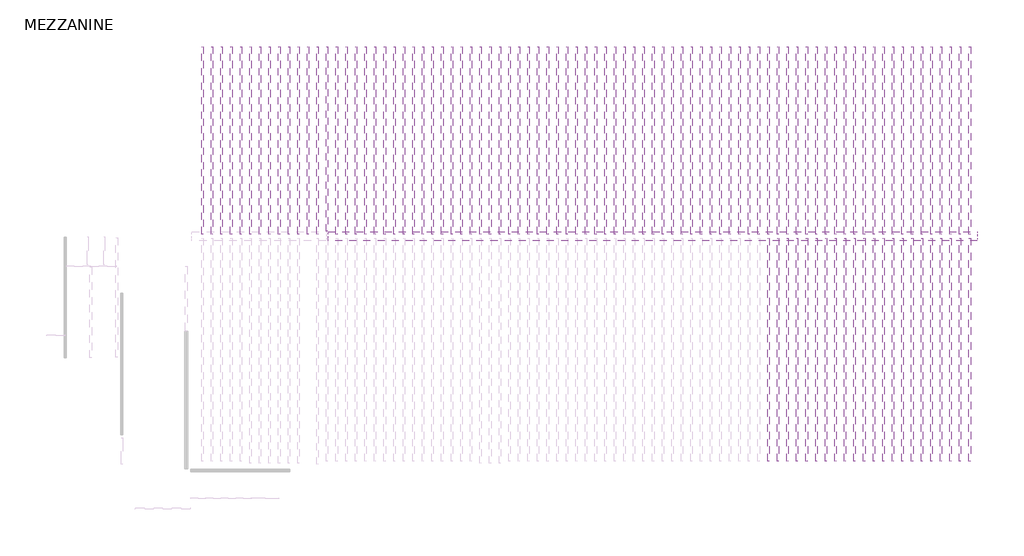
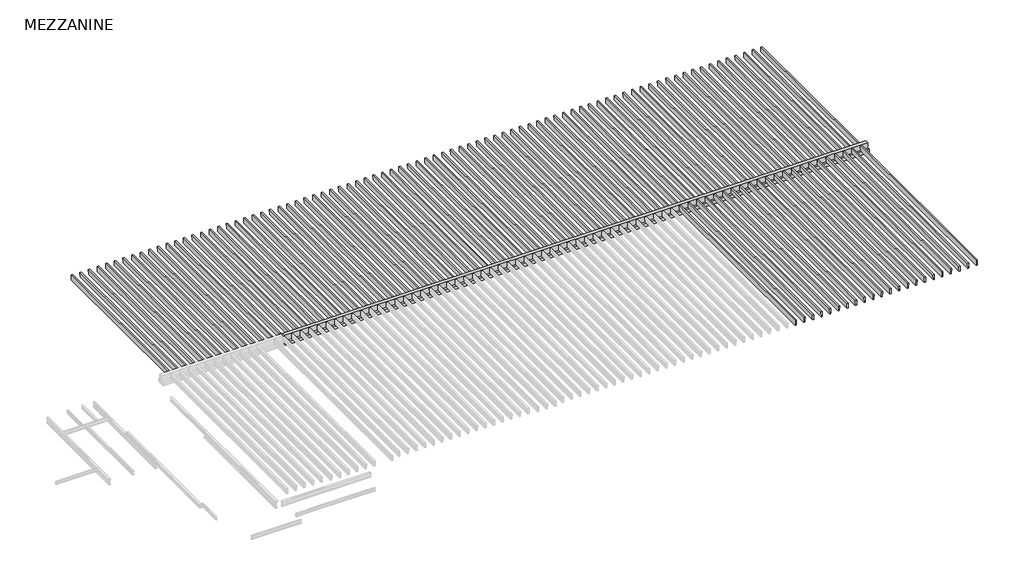
# One storey, part 2 of 2: 104 beams.
"""IFC4 building model written with IfcOpenShell, lengths in millimetres."""

import ifcopenshell
import ifcopenshell.guid

model = None  # the IFC model being written
_history = None  # IfcOwnerHistory: only IFC2X3 demands one
_inside = {}  # id of a spatial element -> (the spatial element, [elements in it])
_under = {}  # id of a project, library or spatial element -> (it, [spatial elements below it])
_declared = {}  # id of a project -> (the project, [libraries it declares])
_typed = {}  # id of a type object -> (the type object, [elements of that type])
_made_of = {}  # id of a material, layer set ... -> (it, [elements and type objects made of it])


def new_model(schema):
    """Start an empty IFC model of exactly this schema.

    Asked for "IFC4X3", IfcOpenShell would pick the latest addendum, in which some entities
    have other attributes; the version numbers below select the first issue.
    IFC2X3 requires an IfcOwnerHistory on every rooted entity: one is made here for all.
    """
    global model, _history
    if schema == "IFC4X3":
        model = ifcopenshell.file(schema_version=(4, 3, 0, 0))
    else:
        model = ifcopenshell.file(schema=schema)
    _inside.clear()
    _under.clear()
    _declared.clear()
    _typed.clear()
    _made_of.clear()
    _history = None
    if model.schema == "IFC2X3":
        org = make("IfcOrganization", Name="unknown")
        user = make(
            "IfcPersonAndOrganization",
            ThePerson=make("IfcPerson", FamilyName="unknown"),
            TheOrganization=org,
        )
        app = make(
            "IfcApplication",
            ApplicationDeveloper=org,
            Version="unknown",
            ApplicationFullName="unknown",
            ApplicationIdentifier="unknown",
        )
        _history = make(
            "IfcOwnerHistory",
            OwningUser=user,
            OwningApplication=app,
            ChangeAction="ADDED",
            CreationDate=0,
        )
    return model


def make(cls, **values):
    """One entity of the class cls with the attributes given. An attribute that is None is left unset."""
    return model.create_entity(
        cls, **{name: value for name, value in values.items() if value is not None}
    )


def rooted(cls, **values):
    """An entity with a GlobalId (a new one), such as an element, a storey or a relation."""
    return make(cls, GlobalId=ifcopenshell.guid.new(), OwnerHistory=_history, **values)


def si_unit(unit_type, name, prefix=None):
    """IfcSIUnit, for example si_unit("LENGTHUNIT", "METRE", prefix="MILLI")."""
    return make("IfcSIUnit", UnitType=unit_type, Prefix=prefix, Name=name)


def assignment(units):
    """IfcUnitAssignment: the units of a project."""
    return None if units is None else make("IfcUnitAssignment", Units=units)


def point(xyz):
    """IfcCartesianPoint."""
    return None if xyz is None else make("IfcCartesianPoint", Coordinates=xyz)


def direction(xyz):
    """IfcDirection."""
    return None if xyz is None else make("IfcDirection", DirectionRatios=xyz)


def frame(location, z_axis=None, x_axis=None):
    """IfcAxis2Placement3D, a coordinate frame: its origin and axes. An axis left out is left unset."""
    return make(
        "IfcAxis2Placement3D",
        Location=point(location),
        Axis=direction(z_axis),
        RefDirection=direction(x_axis),
    )


def origin():
    """The frame at (0, 0, 0) with its axes left unset."""
    return frame((0.0, 0.0, 0.0))


def place(relative_to, where):
    """IfcLocalPlacement: puts the frame where relative to a parent placement (None: the world)."""
    return make(
        "IfcLocalPlacement", PlacementRelTo=relative_to, RelativePlacement=where
    )


def context(
    kind, dimensions, precision=None, world=None, true_north=None, identifier=None
):
    """IfcGeometricRepresentationContext, for example the 3D "Model" context."""
    return make(
        "IfcGeometricRepresentationContext",
        ContextIdentifier=identifier,
        ContextType=kind,
        CoordinateSpaceDimension=dimensions,
        Precision=precision,
        WorldCoordinateSystem=world,
        TrueNorth=true_north,
    )


def project(units=None, contexts=None):
    """IfcProject with its units and contexts."""
    return rooted(
        "IfcProject",
        Name="project",
        RepresentationContexts=contexts,
        UnitsInContext=assignment(units),
    )


def spatial(cls, under=None, at=None, **own):
    """A site, building, storey or space (cls), placed at a placement, below another one or the project."""
    s = rooted(cls, ObjectPlacement=at, **own)
    if under is not None:
        _under.setdefault(under.id(), (under, []))[1].append(s)
    return s


def polyline(points):
    """IfcPolyline through the points."""
    return make("IfcPolyline", Points=[point(p) for p in points])


def outline(outer, holes=None, kind="AREA"):
    """IfcArbitraryClosedProfileDef: a profile drawn as a closed curve; with holes, ...WithVoids."""
    if holes is None:
        return make("IfcArbitraryClosedProfileDef", ProfileType=kind, OuterCurve=outer)
    return make(
        "IfcArbitraryProfileDefWithVoids",
        ProfileType=kind,
        OuterCurve=outer,
        InnerCurves=holes,
    )


def extrude(swept, where, along, depth):
    """IfcExtrudedAreaSolid: the profile swept, set in the frame where, extruded along a direction by depth."""
    return make(
        "IfcExtrudedAreaSolid",
        SweptArea=swept,
        Position=where,
        ExtrudedDirection=direction(along),
        Depth=depth,
    )


def shape(context_of_items, identifier, shape_type, items):
    """IfcShapeRepresentation: the items that make up one representation, for example the "Body"."""
    return make(
        "IfcShapeRepresentation",
        ContextOfItems=context_of_items,
        RepresentationIdentifier=identifier,
        RepresentationType=shape_type,
        Items=items,
    )


def source(mapping_origin, context_of_items, identifier, shape_type, items):
    """IfcRepresentationMap: a shape defined once, which mapped items show again and again."""
    return make(
        "IfcRepresentationMap",
        MappingOrigin=mapping_origin,
        MappedRepresentation=shape(context_of_items, identifier, shape_type, items),
    )


def transform(
    local_origin,
    x_axis=None,
    y_axis=None,
    z_axis=None,
    scale=None,
    scale2=None,
    scale3=None,
    uniform=True,
):
    """IfcCartesianTransformationOperator3D, or its non-uniform kind. x_axis, y_axis, z_axis: its Axis1, 2, 3."""
    if uniform:
        return make(
            "IfcCartesianTransformationOperator3D",
            Axis1=direction(x_axis),
            Axis2=direction(y_axis),
            LocalOrigin=point(local_origin),
            Scale=scale,
            Axis3=direction(z_axis),
        )
    return make(
        "IfcCartesianTransformationOperator3DnonUniform",
        Axis1=direction(x_axis),
        Axis2=direction(y_axis),
        LocalOrigin=point(local_origin),
        Scale=scale,
        Axis3=direction(z_axis),
        Scale2=scale2,
        Scale3=scale3,
    )


def mapped(mapping_source, mapping_target):
    """IfcMappedItem: shows the shape of a source again, moved by a transform."""
    return make(
        "IfcMappedItem", MappingSource=mapping_source, MappingTarget=mapping_target
    )


def made_of(thing, what):
    """Note that an element or type object is made of a material, layer set ...; save() writes the relation."""
    if what is not None:
        _made_of.setdefault(what.id(), (what, []))[1].append(thing)
    return thing


def element(
    cls,
    number,
    at=None,
    inside=None,
    cuts=None,
    type_object=None,
    material=None,
    context=None,
    identifier="Body",
    shape_type=None,
    held_by="IfcProductDefinitionShape",
    body=None,
    shapes=None,
    **own,
):
    """One element of the class cls, such as IfcWall. Its Tag is "e" and its number.

    at: its placement. inside: the storey or other place that contains it. cuts: it is an
    opening in that element (IfcRelVoidsElement). A single representation is given by context,
    identifier, shape_type and body (its items); several are given by shapes. held_by: the class
    of the entity that holds the representations. save() writes the other relations.
    """
    e = rooted(cls, Tag="e%d" % number, ObjectPlacement=at, **own)
    if body is not None:
        shapes = [shape(context, identifier, shape_type, body)]
    if shapes is not None:
        e.Representation = make(held_by, Representations=shapes)
    if inside is not None:
        _inside.setdefault(inside.id(), (inside, []))[1].append(e)
    if cuts is not None:
        rooted(
            "IfcRelVoidsElement", RelatingBuildingElement=cuts, RelatedOpeningElement=e
        )
    if type_object is not None:
        _typed.setdefault(type_object.id(), (type_object, []))[1].append(e)
    return made_of(e, material)


def aggregate(whole, parts):
    """IfcRelAggregates: a whole, such as a stair, and the parts it consists of."""
    return rooted("IfcRelAggregates", RelatingObject=whole, RelatedObjects=parts)


def save(model, path):
    """Write the relations noted so far, then the file.

    IfcRelAggregates (storeys below a building ...), IfcRelContainedInSpatialStructure (elements
    in a storey), IfcRelDefinesByType, IfcRelAssociatesMaterial and IfcRelDeclares: one each for
    every whole, place, type object, material and project.
    """
    for whole, parts in _under.values():
        aggregate(whole, parts)
    for where, things in _inside.values():
        rooted(
            "IfcRelContainedInSpatialStructure",
            RelatedElements=things,
            RelatingStructure=where,
        )
    for kind, things in _typed.values():
        rooted("IfcRelDefinesByType", RelatedObjects=things, RelatingType=kind)
    for what, things in _made_of.values():
        rooted("IfcRelAssociatesMaterial", RelatedObjects=things, RelatingMaterial=what)
    for by, libraries in _declared.values():
        rooted("IfcRelDeclares", RelatingContext=by, RelatedDefinitions=libraries)
    model.write(path)


def precast_cone_shaped_beam_double_t_c0c18137(model_context):
    return source(origin(), model_context, "Body", "SweptSolid", [
        extrude(outline(polyline([(50.8, -228.6), (-50.8, -228.6), (-63.5, 228.6), (63.5, 228.6), (50.8, -228.6)])), frame((-7378.7, 0.0, 0.0), z_axis=(1.0, 0.0, 0.0), x_axis=(0.0, 1.0, 0.0)), (0.0, 0.0, 1.0), 14909.8),
    ])


def precast_cone_shaped_beam_double_t_e9a1f935(model_context):
    return source(origin(), model_context, "Body", "SweptSolid", [
        extrude(outline(polyline([(50.8, -228.6), (-50.8, -228.6), (-63.5, 228.6), (63.5, 228.6), (50.8, -228.6)])), frame((-7162.8, 0.0, 0.0), z_axis=(1.0, 0.0, 0.0), x_axis=(0.0, 1.0, 0.0)), (0.0, 0.0, 1.0), 14693.9),
    ])


def precast_cone_shaped_beam_double_t_b6a0bb25(model_context):
    return source(origin(), model_context, "Body", "SweptSolid", [
        extrude(outline(polyline([(-50.8, -228.6), (-63.5, 228.6), (63.5, 228.6), (50.8, -228.6), (-50.8, -228.6)])), frame((-8915.4, 0.0, 0.0), z_axis=(1.0, 0.0, 0.0), x_axis=(0.0, 1.0, 0.0)), (0.0, 0.0, 1.0), 17741.9),
    ])


def precast_inverted_tee_20_12x28_ea35af0b(model_context):
    return source(origin(), model_context, "Body", "SweptSolid", [
        extrude(outline(polyline([(-355.6, -406.4), (-355.6, -101.6), (-152.4, -101.6), (-152.4, 406.4), (152.4, 406.4), (152.4, -101.6), (355.6, -101.6), (355.6, -406.4), (-355.6, -406.4)])), frame((-25831.8, 0.0, 0.0), z_axis=(1.0, 0.0, 0.0), x_axis=(0.0, 1.0, 0.0)), (0.0, 0.0, 1.0), 51587.4),
    ])


model = new_model("IFC4")

# Units and contexts
model_context = context("Model", 3, world=origin())
ifc_project = project(units=[si_unit("LENGTHUNIT", "METRE", prefix="MILLI")], contexts=[model_context])

# Site, building, storey
site = spatial("IfcSite", under=ifc_project)
building = spatial("IfcBuilding", under=site)
storey = spatial("IfcBuildingStorey", under=building, Name="MEZZANINE", Elevation=2959.1)

# Beams
placement = place(None, origin())
precast_cone_shaped_beam_double_t_shape = precast_cone_shaped_beam_double_t_c0c18137(model_context)
element("IfcBeam", 1, ObjectType="Precast-Cone Shaped Beam : DOUBLE_T", at=placement, inside=storey, context=model_context, shape_type="MappedRepresentation", body=[
    mapped(precast_cone_shaped_beam_double_t_shape, transform((-23461.5909443, 5367.0768471, 4724.4), x_axis=(0.0, 1.0, 0.0), y_axis=(-1.0, 0.0, 0.0), z_axis=(0.0, 0.0, 1.0))),
])
element("IfcBeam", 2, ObjectType="Precast-Cone Shaped Beam : DOUBLE_T", at=placement, inside=storey, context=model_context, shape_type="MappedRepresentation", body=[
    mapped(precast_cone_shaped_beam_double_t_shape, transform((-22699.5909443, 5367.0768471, 4724.4), x_axis=(0.0, 1.0, 0.0), y_axis=(-1.0, 0.0, 0.0), z_axis=(0.0, 0.0, 1.0))),
])
element("IfcBeam", 3, ObjectType="Precast-Cone Shaped Beam : DOUBLE_T", at=placement, inside=storey, context=model_context, shape_type="MappedRepresentation", body=[
    mapped(precast_cone_shaped_beam_double_t_shape, transform((-21937.5909443, 5367.0768471, 4724.4), x_axis=(0.0, 1.0, 0.0), y_axis=(-1.0, 0.0, 0.0), z_axis=(0.0, 0.0, 1.0))),
])
element("IfcBeam", 4, ObjectType="Precast-Cone Shaped Beam : DOUBLE_T", at=placement, inside=storey, context=model_context, shape_type="MappedRepresentation", body=[
    mapped(precast_cone_shaped_beam_double_t_shape, transform((-21175.5909443, 5367.0768471, 4724.4), x_axis=(0.0, 1.0, 0.0), y_axis=(-1.0, 0.0, 0.0), z_axis=(0.0, 0.0, 1.0))),
])
element("IfcBeam", 5, ObjectType="Precast-Cone Shaped Beam : DOUBLE_T", at=placement, inside=storey, context=model_context, shape_type="MappedRepresentation", body=[
    mapped(precast_cone_shaped_beam_double_t_shape, transform((-20413.5909443, 5367.0768471, 4724.4), x_axis=(0.0, 1.0, 0.0), y_axis=(-1.0, 0.0, 0.0), z_axis=(0.0, 0.0, 1.0))),
])
element("IfcBeam", 6, ObjectType="Precast-Cone Shaped Beam : DOUBLE_T", at=placement, inside=storey, context=model_context, shape_type="MappedRepresentation", body=[
    mapped(precast_cone_shaped_beam_double_t_shape, transform((-19651.5909443, 5367.0768471, 4724.4), x_axis=(0.0, 1.0, 0.0), y_axis=(-1.0, 0.0, 0.0), z_axis=(0.0, 0.0, 1.0))),
])
element("IfcBeam", 7, ObjectType="Precast-Cone Shaped Beam : DOUBLE_T", at=placement, inside=storey, context=model_context, shape_type="MappedRepresentation", body=[
    mapped(precast_cone_shaped_beam_double_t_shape, transform((-18889.5909443, 5367.0768471, 4724.4), x_axis=(0.0, 1.0, 0.0), y_axis=(-1.0, 0.0, 0.0), z_axis=(0.0, 0.0, 1.0))),
])
element("IfcBeam", 8, ObjectType="Precast-Cone Shaped Beam : DOUBLE_T", at=placement, inside=storey, context=model_context, shape_type="MappedRepresentation", body=[
    mapped(precast_cone_shaped_beam_double_t_shape, transform((-18127.5909443, 5367.0768471, 4724.4), x_axis=(0.0, 1.0, 0.0), y_axis=(-1.0, 0.0, 0.0), z_axis=(0.0, 0.0, 1.0))),
])
element("IfcBeam", 9, ObjectType="Precast-Cone Shaped Beam : DOUBLE_T", at=placement, inside=storey, context=model_context, shape_type="MappedRepresentation", body=[
    mapped(precast_cone_shaped_beam_double_t_shape, transform((-17365.5909443, 5367.0768471, 4724.4), x_axis=(0.0, 1.0, 0.0), y_axis=(-1.0, 0.0, 0.0), z_axis=(0.0, 0.0, 1.0))),
])
element("IfcBeam", 10, ObjectType="Precast-Cone Shaped Beam : DOUBLE_T", at=placement, inside=storey, context=model_context, shape_type="MappedRepresentation", body=[
    mapped(precast_cone_shaped_beam_double_t_shape, transform((-16603.5909443, 5367.0768471, 4724.4), x_axis=(0.0, 1.0, 0.0), y_axis=(-1.0, 0.0, 0.0), z_axis=(0.0, 0.0, 1.0))),
])
element("IfcBeam", 11, ObjectType="Precast-Cone Shaped Beam : DOUBLE_T", at=placement, inside=storey, context=model_context, shape_type="MappedRepresentation", body=[
    mapped(precast_cone_shaped_beam_double_t_shape, transform((-15841.5909443, 5367.0768471, 4724.4), x_axis=(0.0, 1.0, 0.0), y_axis=(-1.0, 0.0, 0.0), z_axis=(0.0, 0.0, 1.0))),
])
element("IfcBeam", 12, ObjectType="Precast-Cone Shaped Beam : DOUBLE_T", at=placement, inside=storey, context=model_context, shape_type="MappedRepresentation", body=[
    mapped(precast_cone_shaped_beam_double_t_shape, transform((-15079.5909443, 5367.0768471, 4724.4), x_axis=(0.0, 1.0, 0.0), y_axis=(-1.0, 0.0, 0.0), z_axis=(0.0, 0.0, 1.0))),
])
element("IfcBeam", 13, ObjectType="Precast-Cone Shaped Beam : DOUBLE_T", at=placement, inside=storey, context=model_context, shape_type="MappedRepresentation", body=[
    mapped(precast_cone_shaped_beam_double_t_shape, transform((-14317.5909443, 5367.0768471, 4724.4), x_axis=(0.0, 1.0, 0.0), y_axis=(-1.0, 0.0, 0.0), z_axis=(0.0, 0.0, 1.0))),
])
element("IfcBeam", 14, ObjectType="Precast-Cone Shaped Beam : DOUBLE_T", at=placement, inside=storey, context=model_context, shape_type="MappedRepresentation", body=[
    mapped(precast_cone_shaped_beam_double_t_shape, transform((-13555.5909443, 5367.0768471, 4724.4), x_axis=(0.0, 1.0, 0.0), y_axis=(-1.0, 0.0, 0.0), z_axis=(0.0, 0.0, 1.0))),
])
element("IfcBeam", 15, ObjectType="Precast-Cone Shaped Beam : DOUBLE_T", at=placement, inside=storey, context=model_context, shape_type="MappedRepresentation", body=[
    mapped(precast_cone_shaped_beam_double_t_shape, transform((-12793.5909443, 5367.0768471, 4724.4), x_axis=(0.0, 1.0, 0.0), y_axis=(-1.0, 0.0, 0.0), z_axis=(0.0, 0.0, 1.0))),
])
element("IfcBeam", 16, ObjectType="Precast-Cone Shaped Beam : DOUBLE_T", at=placement, inside=storey, context=model_context, shape_type="MappedRepresentation", body=[
    mapped(precast_cone_shaped_beam_double_t_shape, transform((-12031.5909443, 5367.0768471, 4724.4), x_axis=(0.0, 1.0, 0.0), y_axis=(-1.0, 0.0, 0.0), z_axis=(0.0, 0.0, 1.0))),
])
element("IfcBeam", 17, ObjectType="Precast-Cone Shaped Beam : DOUBLE_T", at=placement, inside=storey, context=model_context, shape_type="MappedRepresentation", body=[
    mapped(precast_cone_shaped_beam_double_t_shape, transform((-11269.5909443, 5367.0768471, 4724.4), x_axis=(0.0, 1.0, 0.0), y_axis=(-1.0, 0.0, 0.0), z_axis=(0.0, 0.0, 1.0))),
])
element("IfcBeam", 18, ObjectType="Precast-Cone Shaped Beam : DOUBLE_T", at=placement, inside=storey, context=model_context, shape_type="MappedRepresentation", body=[
    mapped(precast_cone_shaped_beam_double_t_shape, transform((-10507.5909443, 5367.0768471, 4724.4), x_axis=(0.0, 1.0, 0.0), y_axis=(-1.0, 0.0, 0.0), z_axis=(0.0, 0.0, 1.0))),
])
element("IfcBeam", 19, ObjectType="Precast-Cone Shaped Beam : DOUBLE_T", at=placement, inside=storey, context=model_context, shape_type="MappedRepresentation", body=[
    mapped(precast_cone_shaped_beam_double_t_shape, transform((-9745.5909443, 5367.0768471, 4724.4), x_axis=(0.0, 1.0, 0.0), y_axis=(-1.0, 0.0, 0.0), z_axis=(0.0, 0.0, 1.0))),
])
element("IfcBeam", 20, ObjectType="Precast-Cone Shaped Beam : DOUBLE_T", at=placement, inside=storey, context=model_context, shape_type="MappedRepresentation", body=[
    mapped(precast_cone_shaped_beam_double_t_shape, transform((-8983.5909443, 5367.0768471, 4724.4), x_axis=(0.0, 1.0, 0.0), y_axis=(-1.0, 0.0, 0.0), z_axis=(0.0, 0.0, 1.0))),
])
element("IfcBeam", 21, ObjectType="Precast-Cone Shaped Beam : DOUBLE_T", at=placement, inside=storey, context=model_context, shape_type="MappedRepresentation", body=[
    mapped(precast_cone_shaped_beam_double_t_shape, transform((-8221.5909443, 5367.0768471, 4724.4), x_axis=(0.0, 1.0, 0.0), y_axis=(-1.0, 0.0, 0.0), z_axis=(0.0, 0.0, 1.0))),
])
element("IfcBeam", 22, ObjectType="Precast-Cone Shaped Beam : DOUBLE_T", at=placement, inside=storey, context=model_context, shape_type="MappedRepresentation", body=[
    mapped(precast_cone_shaped_beam_double_t_shape, transform((-7459.5909443, 5367.0768471, 4724.4), x_axis=(0.0, 1.0, 0.0), y_axis=(-1.0, 0.0, 0.0), z_axis=(0.0, 0.0, 1.0))),
])
element("IfcBeam", 23, ObjectType="Precast-Cone Shaped Beam : DOUBLE_T", at=placement, inside=storey, context=model_context, shape_type="MappedRepresentation", body=[
    mapped(precast_cone_shaped_beam_double_t_shape, transform((-6697.5909443, 5367.0768471, 4724.4), x_axis=(0.0, 1.0, 0.0), y_axis=(-1.0, 0.0, 0.0), z_axis=(0.0, 0.0, 1.0))),
])
element("IfcBeam", 24, ObjectType="Precast-Cone Shaped Beam : DOUBLE_T", at=placement, inside=storey, context=model_context, shape_type="MappedRepresentation", body=[
    mapped(precast_cone_shaped_beam_double_t_shape, transform((-5935.5909443, 5367.0768471, 4724.4), x_axis=(0.0, 1.0, 0.0), y_axis=(-1.0, 0.0, 0.0), z_axis=(0.0, 0.0, 1.0))),
])
element("IfcBeam", 25, ObjectType="Precast-Cone Shaped Beam : DOUBLE_T", at=placement, inside=storey, context=model_context, shape_type="MappedRepresentation", body=[
    mapped(precast_cone_shaped_beam_double_t_shape, transform((-5173.5909443, 5367.0768471, 4724.4), x_axis=(0.0, 1.0, 0.0), y_axis=(-1.0, 0.0, 0.0), z_axis=(0.0, 0.0, 1.0))),
])
element("IfcBeam", 26, ObjectType="Precast-Cone Shaped Beam : DOUBLE_T", at=placement, inside=storey, context=model_context, shape_type="MappedRepresentation", body=[
    mapped(precast_cone_shaped_beam_double_t_shape, transform((-4411.5909443, 5367.0768471, 4724.4), x_axis=(0.0, 1.0, 0.0), y_axis=(-1.0, 0.0, 0.0), z_axis=(0.0, 0.0, 1.0))),
])
element("IfcBeam", 27, ObjectType="Precast-Cone Shaped Beam : DOUBLE_T", at=placement, inside=storey, context=model_context, shape_type="MappedRepresentation", body=[
    mapped(precast_cone_shaped_beam_double_t_shape, transform((-3649.5909443, 5367.0768471, 4724.4), x_axis=(0.0, 1.0, 0.0), y_axis=(-1.0, 0.0, 0.0), z_axis=(0.0, 0.0, 1.0))),
])
element("IfcBeam", 28, ObjectType="Precast-Cone Shaped Beam : DOUBLE_T", at=placement, inside=storey, context=model_context, shape_type="MappedRepresentation", body=[
    mapped(precast_cone_shaped_beam_double_t_shape, transform((-2887.5909443, 5367.0768471, 4724.4), x_axis=(0.0, 1.0, 0.0), y_axis=(-1.0, 0.0, 0.0), z_axis=(0.0, 0.0, 1.0))),
])
element("IfcBeam", 29, ObjectType="Precast-Cone Shaped Beam : DOUBLE_T", at=placement, inside=storey, context=model_context, shape_type="MappedRepresentation", body=[
    mapped(precast_cone_shaped_beam_double_t_shape, transform((-2125.5909443, 5367.0768471, 4724.4), x_axis=(0.0, 1.0, 0.0), y_axis=(-1.0, 0.0, 0.0), z_axis=(0.0, 0.0, 1.0))),
])
element("IfcBeam", 30, ObjectType="Precast-Cone Shaped Beam : DOUBLE_T", at=placement, inside=storey, context=model_context, shape_type="MappedRepresentation", body=[
    mapped(precast_cone_shaped_beam_double_t_shape, transform((-1363.5909443, 5367.0768471, 4724.4), x_axis=(0.0, 1.0, 0.0), y_axis=(-1.0, 0.0, 0.0), z_axis=(0.0, 0.0, 1.0))),
])
element("IfcBeam", 31, ObjectType="Precast-Cone Shaped Beam : DOUBLE_T", at=placement, inside=storey, context=model_context, shape_type="MappedRepresentation", body=[
    mapped(precast_cone_shaped_beam_double_t_shape, transform((-601.5909443, 5367.0768471, 4724.4), x_axis=(0.0, 1.0, 0.0), y_axis=(-1.0, 0.0, 0.0), z_axis=(0.0, 0.0, 1.0))),
])
element("IfcBeam", 32, ObjectType="Precast-Cone Shaped Beam : DOUBLE_T", at=placement, inside=storey, context=model_context, shape_type="MappedRepresentation", body=[
    mapped(precast_cone_shaped_beam_double_t_shape, transform((160.4090557, 5367.0768471, 4724.4), x_axis=(0.0, 1.0, 0.0), y_axis=(-1.0, 0.0, 0.0), z_axis=(0.0, 0.0, 1.0))),
])
element("IfcBeam", 33, ObjectType="Precast-Cone Shaped Beam : DOUBLE_T", at=placement, inside=storey, context=model_context, shape_type="MappedRepresentation", body=[
    mapped(precast_cone_shaped_beam_double_t_shape, transform((922.4090557, 5367.0768471, 4724.4), x_axis=(0.0, 1.0, 0.0), y_axis=(-1.0, 0.0, 0.0), z_axis=(0.0, 0.0, 1.0))),
])
element("IfcBeam", 34, ObjectType="Precast-Cone Shaped Beam : DOUBLE_T", at=placement, inside=storey, context=model_context, shape_type="MappedRepresentation", body=[
    mapped(precast_cone_shaped_beam_double_t_shape, transform((1684.4090557, 5367.0768471, 4724.4), x_axis=(0.0, 1.0, 0.0), y_axis=(-1.0, 0.0, 0.0), z_axis=(0.0, 0.0, 1.0))),
])
element("IfcBeam", 35, ObjectType="Precast-Cone Shaped Beam : DOUBLE_T", at=placement, inside=storey, context=model_context, shape_type="MappedRepresentation", body=[
    mapped(precast_cone_shaped_beam_double_t_shape, transform((2446.4090557, 5367.0768471, 4724.4), x_axis=(0.0, 1.0, 0.0), y_axis=(-1.0, 0.0, 0.0), z_axis=(0.0, 0.0, 1.0))),
])
element("IfcBeam", 36, ObjectType="Precast-Cone Shaped Beam : DOUBLE_T", at=placement, inside=storey, context=model_context, shape_type="MappedRepresentation", body=[
    mapped(precast_cone_shaped_beam_double_t_shape, transform((3208.4090557, 5367.0768471, 4724.4), x_axis=(0.0, 1.0, 0.0), y_axis=(-1.0, 0.0, 0.0), z_axis=(0.0, 0.0, 1.0))),
])
element("IfcBeam", 37, ObjectType="Precast-Cone Shaped Beam : DOUBLE_T", at=placement, inside=storey, context=model_context, shape_type="MappedRepresentation", body=[
    mapped(precast_cone_shaped_beam_double_t_shape, transform((3970.4090557, 5367.0768471, 4724.4), x_axis=(0.0, 1.0, 0.0), y_axis=(-1.0, 0.0, 0.0), z_axis=(0.0, 0.0, 1.0))),
])
element("IfcBeam", 38, ObjectType="Precast-Cone Shaped Beam : DOUBLE_T", at=placement, inside=storey, context=model_context, shape_type="MappedRepresentation", body=[
    mapped(precast_cone_shaped_beam_double_t_shape, transform((4732.4090557, 5367.0768471, 4724.4), x_axis=(0.0, 1.0, 0.0), y_axis=(-1.0, 0.0, 0.0), z_axis=(0.0, 0.0, 1.0))),
])
element("IfcBeam", 39, ObjectType="Precast-Cone Shaped Beam : DOUBLE_T", at=placement, inside=storey, context=model_context, shape_type="MappedRepresentation", body=[
    mapped(precast_cone_shaped_beam_double_t_shape, transform((5494.4090557, 5367.0768471, 4724.4), x_axis=(0.0, 1.0, 0.0), y_axis=(-1.0, 0.0, 0.0), z_axis=(0.0, 0.0, 1.0))),
])
element("IfcBeam", 40, ObjectType="Precast-Cone Shaped Beam : DOUBLE_T", at=placement, inside=storey, context=model_context, shape_type="MappedRepresentation", body=[
    mapped(precast_cone_shaped_beam_double_t_shape, transform((6256.4090557, 5367.0768471, 4724.4), x_axis=(0.0, 1.0, 0.0), y_axis=(-1.0, 0.0, 0.0), z_axis=(0.0, 0.0, 1.0))),
])
element("IfcBeam", 41, ObjectType="Precast-Cone Shaped Beam : DOUBLE_T", at=placement, inside=storey, context=model_context, shape_type="MappedRepresentation", body=[
    mapped(precast_cone_shaped_beam_double_t_shape, transform((7018.4090557, 5367.0768471, 4724.4), x_axis=(0.0, 1.0, 0.0), y_axis=(-1.0, 0.0, 0.0), z_axis=(0.0, 0.0, 1.0))),
])
element("IfcBeam", 42, ObjectType="Precast-Cone Shaped Beam : DOUBLE_T", at=placement, inside=storey, context=model_context, shape_type="MappedRepresentation", body=[
    mapped(precast_cone_shaped_beam_double_t_shape, transform((7780.4090557, 5367.0768471, 4724.4), x_axis=(0.0, 1.0, 0.0), y_axis=(-1.0, 0.0, 0.0), z_axis=(0.0, 0.0, 1.0))),
])
element("IfcBeam", 43, ObjectType="Precast-Cone Shaped Beam : DOUBLE_T", at=placement, inside=storey, context=model_context, shape_type="MappedRepresentation", body=[
    mapped(precast_cone_shaped_beam_double_t_shape, transform((8542.4090557, 5367.0768471, 4724.4), x_axis=(0.0, 1.0, 0.0), y_axis=(-1.0, 0.0, 0.0), z_axis=(0.0, 0.0, 1.0))),
])
element("IfcBeam", 44, ObjectType="Precast-Cone Shaped Beam : DOUBLE_T", at=placement, inside=storey, context=model_context, shape_type="MappedRepresentation", body=[
    mapped(precast_cone_shaped_beam_double_t_shape, transform((9304.4090557, 5367.0768471, 4724.4), x_axis=(0.0, 1.0, 0.0), y_axis=(-1.0, 0.0, 0.0), z_axis=(0.0, 0.0, 1.0))),
])
element("IfcBeam", 45, ObjectType="Precast-Cone Shaped Beam : DOUBLE_T", at=placement, inside=storey, context=model_context, shape_type="MappedRepresentation", body=[
    mapped(precast_cone_shaped_beam_double_t_shape, transform((10066.4090557, 5367.0768471, 4724.4), x_axis=(0.0, 1.0, 0.0), y_axis=(-1.0, 0.0, 0.0), z_axis=(0.0, 0.0, 1.0))),
])
element("IfcBeam", 46, ObjectType="Precast-Cone Shaped Beam : DOUBLE_T", at=placement, inside=storey, context=model_context, shape_type="MappedRepresentation", body=[
    mapped(precast_cone_shaped_beam_double_t_shape, transform((10828.4090557, 5367.0768471, 4724.4), x_axis=(0.0, 1.0, 0.0), y_axis=(-1.0, 0.0, 0.0), z_axis=(0.0, 0.0, 1.0))),
])
element("IfcBeam", 47, ObjectType="Precast-Cone Shaped Beam : DOUBLE_T", at=placement, inside=storey, context=model_context, shape_type="MappedRepresentation", body=[
    mapped(precast_cone_shaped_beam_double_t_shape, transform((11590.4090557, 5367.0768471, 4724.4), x_axis=(0.0, 1.0, 0.0), y_axis=(-1.0, 0.0, 0.0), z_axis=(0.0, 0.0, 1.0))),
])
element("IfcBeam", 48, ObjectType="Precast-Cone Shaped Beam : DOUBLE_T", at=placement, inside=storey, context=model_context, shape_type="MappedRepresentation", body=[
    mapped(precast_cone_shaped_beam_double_t_shape, transform((12352.4090557, 5367.0768471, 4724.4), x_axis=(0.0, 1.0, 0.0), y_axis=(-1.0, 0.0, 0.0), z_axis=(0.0, 0.0, 1.0))),
])
element("IfcBeam", 49, ObjectType="Precast-Cone Shaped Beam : DOUBLE_T", at=placement, inside=storey, context=model_context, shape_type="MappedRepresentation", body=[
    mapped(precast_cone_shaped_beam_double_t_shape, transform((13114.4090557, 5367.0768471, 4724.4), x_axis=(0.0, 1.0, 0.0), y_axis=(-1.0, 0.0, 0.0), z_axis=(0.0, 0.0, 1.0))),
])
element("IfcBeam", 50, ObjectType="Precast-Cone Shaped Beam : DOUBLE_T", at=placement, inside=storey, context=model_context, shape_type="MappedRepresentation", body=[
    mapped(precast_cone_shaped_beam_double_t_shape, transform((13876.4090557, 5367.0768471, 4724.4), x_axis=(0.0, 1.0, 0.0), y_axis=(-1.0, 0.0, 0.0), z_axis=(0.0, 0.0, 1.0))),
])
element("IfcBeam", 51, ObjectType="Precast-Cone Shaped Beam : DOUBLE_T", at=placement, inside=storey, context=model_context, shape_type="MappedRepresentation", body=[
    mapped(precast_cone_shaped_beam_double_t_shape, transform((14638.4090557, 5367.0768471, 4724.4), x_axis=(0.0, 1.0, 0.0), y_axis=(-1.0, 0.0, 0.0), z_axis=(0.0, 0.0, 1.0))),
])
element("IfcBeam", 52, ObjectType="Precast-Cone Shaped Beam : DOUBLE_T", at=placement, inside=storey, context=model_context, shape_type="MappedRepresentation", body=[
    mapped(precast_cone_shaped_beam_double_t_shape, transform((15400.4090557, 5367.0768471, 4724.4), x_axis=(0.0, 1.0, 0.0), y_axis=(-1.0, 0.0, 0.0), z_axis=(0.0, 0.0, 1.0))),
])
element("IfcBeam", 53, ObjectType="Precast-Cone Shaped Beam : DOUBLE_T", at=placement, inside=storey, context=model_context, shape_type="MappedRepresentation", body=[
    mapped(precast_cone_shaped_beam_double_t_shape, transform((16162.4090557, 5367.0768471, 4724.4), x_axis=(0.0, 1.0, 0.0), y_axis=(-1.0, 0.0, 0.0), z_axis=(0.0, 0.0, 1.0))),
])
element("IfcBeam", 54, ObjectType="Precast-Cone Shaped Beam : DOUBLE_T", at=placement, inside=storey, context=model_context, shape_type="MappedRepresentation", body=[
    mapped(precast_cone_shaped_beam_double_t_shape, transform((16924.4090557, 5367.0768471, 4724.4), x_axis=(0.0, 1.0, 0.0), y_axis=(-1.0, 0.0, 0.0), z_axis=(0.0, 0.0, 1.0))),
])
element("IfcBeam", 55, ObjectType="Precast-Cone Shaped Beam : DOUBLE_T", at=placement, inside=storey, context=model_context, shape_type="MappedRepresentation", body=[
    mapped(precast_cone_shaped_beam_double_t_shape, transform((17686.4090557, 5367.0768471, 4724.4), x_axis=(0.0, 1.0, 0.0), y_axis=(-1.0, 0.0, 0.0), z_axis=(0.0, 0.0, 1.0))),
])
element("IfcBeam", 56, ObjectType="Precast-Cone Shaped Beam : DOUBLE_T", at=placement, inside=storey, context=model_context, shape_type="MappedRepresentation", body=[
    mapped(precast_cone_shaped_beam_double_t_shape, transform((18448.4090557, 5367.0768471, 4724.4), x_axis=(0.0, 1.0, 0.0), y_axis=(-1.0, 0.0, 0.0), z_axis=(0.0, 0.0, 1.0))),
])
element("IfcBeam", 57, ObjectType="Precast-Cone Shaped Beam : DOUBLE_T", at=placement, inside=storey, context=model_context, shape_type="MappedRepresentation", body=[
    mapped(precast_cone_shaped_beam_double_t_shape, transform((19210.4090557, 5367.0768471, 4724.4), x_axis=(0.0, 1.0, 0.0), y_axis=(-1.0, 0.0, 0.0), z_axis=(0.0, 0.0, 1.0))),
])
element("IfcBeam", 58, ObjectType="Precast-Cone Shaped Beam : DOUBLE_T", at=placement, inside=storey, context=model_context, shape_type="MappedRepresentation", body=[
    mapped(precast_cone_shaped_beam_double_t_shape, transform((19972.4090557, 5367.0768471, 4724.4), x_axis=(0.0, 1.0, 0.0), y_axis=(-1.0, 0.0, 0.0), z_axis=(0.0, 0.0, 1.0))),
])
element("IfcBeam", 59, ObjectType="Precast-Cone Shaped Beam : DOUBLE_T", at=placement, inside=storey, context=model_context, shape_type="MappedRepresentation", body=[
    mapped(precast_cone_shaped_beam_double_t_shape, transform((20734.4090557, 5367.0768471, 4724.4), x_axis=(0.0, 1.0, 0.0), y_axis=(-1.0, 0.0, 0.0), z_axis=(0.0, 0.0, 1.0))),
])
element("IfcBeam", 60, ObjectType="Precast-Cone Shaped Beam : DOUBLE_T", at=placement, inside=storey, context=model_context, shape_type="MappedRepresentation", body=[
    mapped(precast_cone_shaped_beam_double_t_shape, transform((21496.4090557, 5367.0768471, 4724.4), x_axis=(0.0, 1.0, 0.0), y_axis=(-1.0, 0.0, 0.0), z_axis=(0.0, 0.0, 1.0))),
])
element("IfcBeam", 61, ObjectType="Precast-Cone Shaped Beam : DOUBLE_T", at=placement, inside=storey, context=model_context, shape_type="MappedRepresentation", body=[
    mapped(precast_cone_shaped_beam_double_t_shape, transform((22258.4090557, 5367.0768471, 4724.4), x_axis=(0.0, 1.0, 0.0), y_axis=(-1.0, 0.0, 0.0), z_axis=(0.0, 0.0, 1.0))),
])
element("IfcBeam", 62, ObjectType="Precast-Cone Shaped Beam : DOUBLE_T", at=placement, inside=storey, context=model_context, shape_type="MappedRepresentation", body=[
    mapped(precast_cone_shaped_beam_double_t_shape, transform((23020.4090557, 5367.0768471, 4724.4), x_axis=(0.0, 1.0, 0.0), y_axis=(-1.0, 0.0, 0.0), z_axis=(0.0, 0.0, 1.0))),
])
element("IfcBeam", 63, ObjectType="Precast-Cone Shaped Beam : DOUBLE_T", at=placement, inside=storey, context=model_context, shape_type="MappedRepresentation", body=[
    mapped(precast_cone_shaped_beam_double_t_shape, transform((23782.4090557, 5367.0768471, 4724.4), x_axis=(0.0, 1.0, 0.0), y_axis=(-1.0, 0.0, 0.0), z_axis=(0.0, 0.0, 1.0))),
])
element("IfcBeam", 64, ObjectType="Precast-Cone Shaped Beam : DOUBLE_T", at=placement, inside=storey, context=model_context, shape_type="MappedRepresentation", body=[
    mapped(precast_cone_shaped_beam_double_t_shape, transform((24544.4090557, 5367.0768471, 4724.4), x_axis=(0.0, 1.0, 0.0), y_axis=(-1.0, 0.0, 0.0), z_axis=(0.0, 0.0, 1.0))),
])
element("IfcBeam", 65, ObjectType="Precast-Cone Shaped Beam : DOUBLE_T", at=placement, inside=storey, context=model_context, shape_type="MappedRepresentation", body=[
    mapped(precast_cone_shaped_beam_double_t_shape, transform((25306.4090557, 5367.0768471, 4724.4), x_axis=(0.0, 1.0, 0.0), y_axis=(-1.0, 0.0, 0.0), z_axis=(0.0, 0.0, 1.0))),
])
element("IfcBeam", 66, ObjectType="Precast-Cone Shaped Beam : DOUBLE_T", at=placement, inside=storey, context=model_context, shape_type="MappedRepresentation", body=[
    mapped(precast_cone_shaped_beam_double_t_shape, transform((26068.4090557, 5367.0768471, 4724.4), x_axis=(0.0, 1.0, 0.0), y_axis=(-1.0, 0.0, 0.0), z_axis=(0.0, 0.0, 1.0))),
])
element("IfcBeam", 67, ObjectType="Precast-Cone Shaped Beam : DOUBLE_T", at=placement, inside=storey, context=model_context, shape_type="MappedRepresentation", body=[
    mapped(precast_cone_shaped_beam_double_t_shape, transform((26830.4090557, 5367.0768471, 4724.4), x_axis=(0.0, 1.0, 0.0), y_axis=(-1.0, 0.0, 0.0), z_axis=(0.0, 0.0, 1.0))),
])
element("IfcBeam", 68, ObjectType="Precast-Cone Shaped Beam : DOUBLE_T", at=placement, inside=storey, context=model_context, shape_type="MappedRepresentation", body=[
    mapped(precast_cone_shaped_beam_double_t_shape, transform((-24985.5909443, 5367.0768471, 4724.4), x_axis=(0.0, 1.0, 0.0), y_axis=(-1.0, 0.0, 0.0), z_axis=(0.0, 0.0, 1.0))),
])
element("IfcBeam", 69, ObjectType="Precast-Cone Shaped Beam : DOUBLE_T", at=placement, inside=storey, context=model_context, shape_type="MappedRepresentation", body=[
    mapped(precast_cone_shaped_beam_double_t_shape, transform((-25747.5909443, 5367.0768471, 4724.4), x_axis=(0.0, 1.0, 0.0), y_axis=(-1.0, 0.0, 0.0), z_axis=(0.0, 0.0, 1.0))),
])
element("IfcBeam", 70, ObjectType="Precast-Cone Shaped Beam : DOUBLE_T", at=placement, inside=storey, context=model_context, shape_type="MappedRepresentation", body=[
    mapped(precast_cone_shaped_beam_double_t_shape, transform((-26509.5909443, 5367.0768471, 4724.4), x_axis=(0.0, 1.0, 0.0), y_axis=(-1.0, 0.0, 0.0), z_axis=(0.0, 0.0, 1.0))),
])
element("IfcBeam", 71, ObjectType="Precast-Cone Shaped Beam : DOUBLE_T", at=placement, inside=storey, context=model_context, shape_type="MappedRepresentation", body=[
    mapped(precast_cone_shaped_beam_double_t_shape, transform((-27271.5909443, 5367.0768471, 4724.4), x_axis=(0.0, 1.0, 0.0), y_axis=(-1.0, 0.0, 0.0), z_axis=(0.0, 0.0, 1.0))),
])
element("IfcBeam", 72, ObjectType="Precast-Cone Shaped Beam : DOUBLE_T", at=placement, inside=storey, context=model_context, shape_type="MappedRepresentation", body=[
    mapped(precast_cone_shaped_beam_double_t_shape, transform((-28033.5909443, 5367.0768471, 4724.4), x_axis=(0.0, 1.0, 0.0), y_axis=(-1.0, 0.0, 0.0), z_axis=(0.0, 0.0, 1.0))),
])
element("IfcBeam", 73, ObjectType="Precast-Cone Shaped Beam : DOUBLE_T", at=placement, inside=storey, context=model_context, shape_type="MappedRepresentation", body=[
    mapped(precast_cone_shaped_beam_double_t_shape, transform((-28795.5909443, 5367.0768471, 4724.4), x_axis=(0.0, 1.0, 0.0), y_axis=(-1.0, 0.0, 0.0), z_axis=(0.0, 0.0, 1.0))),
])
element("IfcBeam", 74, ObjectType="Precast-Cone Shaped Beam : DOUBLE_T", at=placement, inside=storey, context=model_context, shape_type="MappedRepresentation", body=[
    mapped(precast_cone_shaped_beam_double_t_shape, transform((-29557.5909443, 5367.0768471, 4724.4), x_axis=(0.0, 1.0, 0.0), y_axis=(-1.0, 0.0, 0.0), z_axis=(0.0, 0.0, 1.0))),
])
element("IfcBeam", 75, ObjectType="Precast-Cone Shaped Beam : DOUBLE_T", at=placement, inside=storey, context=model_context, shape_type="MappedRepresentation", body=[
    mapped(precast_cone_shaped_beam_double_t_shape, transform((-30319.5909443, 5367.0768471, 4724.4), x_axis=(0.0, 1.0, 0.0), y_axis=(-1.0, 0.0, 0.0), z_axis=(0.0, 0.0, 1.0))),
])
element("IfcBeam", 76, ObjectType="Precast-Cone Shaped Beam : DOUBLE_T", at=placement, inside=storey, context=model_context, shape_type="MappedRepresentation", body=[
    mapped(precast_cone_shaped_beam_double_t_shape, transform((-31081.5909443, 5367.0768471, 4724.4), x_axis=(0.0, 1.0, 0.0), y_axis=(-1.0, 0.0, 0.0), z_axis=(0.0, 0.0, 1.0))),
])
element("IfcBeam", 77, ObjectType="Precast-Cone Shaped Beam : DOUBLE_T", at=placement, inside=storey, context=model_context, shape_type="MappedRepresentation", body=[
    mapped(precast_cone_shaped_beam_double_t_shape, transform((-31843.5909443, 5367.0768471, 4724.4), x_axis=(0.0, 1.0, 0.0), y_axis=(-1.0, 0.0, 0.0), z_axis=(0.0, 0.0, 1.0))),
])
element("IfcBeam", 78, ObjectType="Precast-Cone Shaped Beam : DOUBLE_T", at=placement, inside=storey, context=model_context, shape_type="MappedRepresentation", body=[
    mapped(precast_cone_shaped_beam_double_t_shape, transform((-32605.5909443, 5367.0768471, 4724.4), x_axis=(0.0, 1.0, 0.0), y_axis=(-1.0, 0.0, 0.0), z_axis=(0.0, 0.0, 1.0))),
])
element("IfcBeam", 79, ObjectType="Precast-Cone Shaped Beam : DOUBLE_T", at=placement, inside=storey, context=model_context, shape_type="MappedRepresentation", body=[
    mapped(precast_cone_shaped_beam_double_t_shape, transform((-33367.5909443, 5367.0768471, 4724.4), x_axis=(0.0, 1.0, 0.0), y_axis=(-1.0, 0.0, 0.0), z_axis=(0.0, 0.0, 1.0))),
])
element("IfcBeam", 80, ObjectType="Precast-Cone Shaped Beam : DOUBLE_T", at=placement, inside=storey, context=model_context, shape_type="MappedRepresentation", body=[
    mapped(precast_cone_shaped_beam_double_t_shape, transform((-34129.5909443, 5367.0768471, 4724.4), x_axis=(0.0, 1.0, 0.0), y_axis=(-1.0, 0.0, 0.0), z_axis=(0.0, 0.0, 1.0))),
])
precast_cone_shaped_beam_double_t_2_shape = precast_cone_shaped_beam_double_t_e9a1f935(model_context)
element("IfcBeam", 81, ObjectType="Precast-Cone Shaped Beam : DOUBLE_T", at=placement, inside=storey, context=model_context, shape_type="MappedRepresentation", body=[
    mapped(precast_cone_shaped_beam_double_t_2_shape, transform((-24223.5909443, 5367.0768471, 4724.4), x_axis=(0.0, 1.0, 0.0), y_axis=(-1.0, 0.0, 0.0), z_axis=(0.0, 0.0, 1.0))),
])
precast_cone_shaped_beam_double_t_3_shape = precast_cone_shaped_beam_double_t_b6a0bb25(model_context)
element("IfcBeam", 82, ObjectType="Precast-Cone Shaped Beam : DOUBLE_T", at=placement, inside=storey, context=model_context, shape_type="MappedRepresentation", body=[
    mapped(precast_cone_shaped_beam_double_t_3_shape, transform((10828.4090557, -11231.8231529, 4724.4), x_axis=(0.0, -1.0, 0.0), y_axis=(1.0, 0.0, 0.0), z_axis=(0.0, 0.0, 1.0))),
])
element("IfcBeam", 83, ObjectType="Precast-Cone Shaped Beam : DOUBLE_T", at=placement, inside=storey, context=model_context, shape_type="MappedRepresentation", body=[
    mapped(precast_cone_shaped_beam_double_t_3_shape, transform((11590.4090557, -11231.8231529, 4724.4), x_axis=(0.0, -1.0, 0.0), y_axis=(1.0, 0.0, 0.0), z_axis=(0.0, 0.0, 1.0))),
])
element("IfcBeam", 84, ObjectType="Precast-Cone Shaped Beam : DOUBLE_T", at=placement, inside=storey, context=model_context, shape_type="MappedRepresentation", body=[
    mapped(precast_cone_shaped_beam_double_t_3_shape, transform((12352.4090557, -11231.8231529, 4724.4), x_axis=(0.0, -1.0, 0.0), y_axis=(1.0, 0.0, 0.0), z_axis=(0.0, 0.0, 1.0))),
])
element("IfcBeam", 85, ObjectType="Precast-Cone Shaped Beam : DOUBLE_T", at=placement, inside=storey, context=model_context, shape_type="MappedRepresentation", body=[
    mapped(precast_cone_shaped_beam_double_t_3_shape, transform((13114.4090557, -11231.8231529, 4724.4), x_axis=(0.0, -1.0, 0.0), y_axis=(1.0, 0.0, 0.0), z_axis=(0.0, 0.0, 1.0))),
])
element("IfcBeam", 86, ObjectType="Precast-Cone Shaped Beam : DOUBLE_T", at=placement, inside=storey, context=model_context, shape_type="MappedRepresentation", body=[
    mapped(precast_cone_shaped_beam_double_t_3_shape, transform((13876.4090557, -11231.8231529, 4724.4), x_axis=(0.0, -1.0, 0.0), y_axis=(1.0, 0.0, 0.0), z_axis=(0.0, 0.0, 1.0))),
])
element("IfcBeam", 87, ObjectType="Precast-Cone Shaped Beam : DOUBLE_T", at=placement, inside=storey, context=model_context, shape_type="MappedRepresentation", body=[
    mapped(precast_cone_shaped_beam_double_t_3_shape, transform((14638.4090557, -11231.8231529, 4724.4), x_axis=(0.0, -1.0, 0.0), y_axis=(1.0, 0.0, 0.0), z_axis=(0.0, 0.0, 1.0))),
])
element("IfcBeam", 88, ObjectType="Precast-Cone Shaped Beam : DOUBLE_T", at=placement, inside=storey, context=model_context, shape_type="MappedRepresentation", body=[
    mapped(precast_cone_shaped_beam_double_t_3_shape, transform((15400.4090557, -11231.8231529, 4724.4), x_axis=(0.0, -1.0, 0.0), y_axis=(1.0, 0.0, 0.0), z_axis=(0.0, 0.0, 1.0))),
])
element("IfcBeam", 89, ObjectType="Precast-Cone Shaped Beam : DOUBLE_T", at=placement, inside=storey, context=model_context, shape_type="MappedRepresentation", body=[
    mapped(precast_cone_shaped_beam_double_t_3_shape, transform((16162.4090557, -11231.8231529, 4724.4), x_axis=(0.0, -1.0, 0.0), y_axis=(1.0, 0.0, 0.0), z_axis=(0.0, 0.0, 1.0))),
])
element("IfcBeam", 90, ObjectType="Precast-Cone Shaped Beam : DOUBLE_T", at=placement, inside=storey, context=model_context, shape_type="MappedRepresentation", body=[
    mapped(precast_cone_shaped_beam_double_t_3_shape, transform((16924.4090557, -11231.8231529, 4724.4), x_axis=(0.0, -1.0, 0.0), y_axis=(1.0, 0.0, 0.0), z_axis=(0.0, 0.0, 1.0))),
])
element("IfcBeam", 91, ObjectType="Precast-Cone Shaped Beam : DOUBLE_T", at=placement, inside=storey, context=model_context, shape_type="MappedRepresentation", body=[
    mapped(precast_cone_shaped_beam_double_t_3_shape, transform((17686.4090557, -11231.8231529, 4724.4), x_axis=(0.0, -1.0, 0.0), y_axis=(1.0, 0.0, 0.0), z_axis=(0.0, 0.0, 1.0))),
])
element("IfcBeam", 92, ObjectType="Precast-Cone Shaped Beam : DOUBLE_T", at=placement, inside=storey, context=model_context, shape_type="MappedRepresentation", body=[
    mapped(precast_cone_shaped_beam_double_t_3_shape, transform((18448.4090557, -11231.8231529, 4724.4), x_axis=(0.0, -1.0, 0.0), y_axis=(1.0, 0.0, 0.0), z_axis=(0.0, 0.0, 1.0))),
])
element("IfcBeam", 93, ObjectType="Precast-Cone Shaped Beam : DOUBLE_T", at=placement, inside=storey, context=model_context, shape_type="MappedRepresentation", body=[
    mapped(precast_cone_shaped_beam_double_t_3_shape, transform((19210.4090557, -11231.8231529, 4724.4), x_axis=(0.0, -1.0, 0.0), y_axis=(1.0, 0.0, 0.0), z_axis=(0.0, 0.0, 1.0))),
])
element("IfcBeam", 94, ObjectType="Precast-Cone Shaped Beam : DOUBLE_T", at=placement, inside=storey, context=model_context, shape_type="MappedRepresentation", body=[
    mapped(precast_cone_shaped_beam_double_t_3_shape, transform((19972.4090557, -11231.8231529, 4724.4), x_axis=(0.0, -1.0, 0.0), y_axis=(1.0, 0.0, 0.0), z_axis=(0.0, 0.0, 1.0))),
])
element("IfcBeam", 95, ObjectType="Precast-Cone Shaped Beam : DOUBLE_T", at=placement, inside=storey, context=model_context, shape_type="MappedRepresentation", body=[
    mapped(precast_cone_shaped_beam_double_t_3_shape, transform((20734.4090557, -11231.8231529, 4724.4), x_axis=(0.0, -1.0, 0.0), y_axis=(1.0, 0.0, 0.0), z_axis=(0.0, 0.0, 1.0))),
])
element("IfcBeam", 96, ObjectType="Precast-Cone Shaped Beam : DOUBLE_T", at=placement, inside=storey, context=model_context, shape_type="MappedRepresentation", body=[
    mapped(precast_cone_shaped_beam_double_t_3_shape, transform((21496.4090557, -11231.8231529, 4724.4), x_axis=(0.0, -1.0, 0.0), y_axis=(1.0, 0.0, 0.0), z_axis=(0.0, 0.0, 1.0))),
])
element("IfcBeam", 97, ObjectType="Precast-Cone Shaped Beam : DOUBLE_T", at=placement, inside=storey, context=model_context, shape_type="MappedRepresentation", body=[
    mapped(precast_cone_shaped_beam_double_t_3_shape, transform((22258.4090557, -11231.8231529, 4724.4), x_axis=(0.0, -1.0, 0.0), y_axis=(1.0, 0.0, 0.0), z_axis=(0.0, 0.0, 1.0))),
])
element("IfcBeam", 98, ObjectType="Precast-Cone Shaped Beam : DOUBLE_T", at=placement, inside=storey, context=model_context, shape_type="MappedRepresentation", body=[
    mapped(precast_cone_shaped_beam_double_t_3_shape, transform((23020.4090557, -11231.8231529, 4724.4), x_axis=(0.0, -1.0, 0.0), y_axis=(1.0, 0.0, 0.0), z_axis=(0.0, 0.0, 1.0))),
])
element("IfcBeam", 99, ObjectType="Precast-Cone Shaped Beam : DOUBLE_T", at=placement, inside=storey, context=model_context, shape_type="MappedRepresentation", body=[
    mapped(precast_cone_shaped_beam_double_t_3_shape, transform((23782.4090557, -11231.8231529, 4724.4), x_axis=(0.0, -1.0, 0.0), y_axis=(1.0, 0.0, 0.0), z_axis=(0.0, 0.0, 1.0))),
])
element("IfcBeam", 100, ObjectType="Precast-Cone Shaped Beam : DOUBLE_T", at=placement, inside=storey, context=model_context, shape_type="MappedRepresentation", body=[
    mapped(precast_cone_shaped_beam_double_t_3_shape, transform((24544.4090557, -11231.8231529, 4724.4), x_axis=(0.0, -1.0, 0.0), y_axis=(1.0, 0.0, 0.0), z_axis=(0.0, 0.0, 1.0))),
])
element("IfcBeam", 101, ObjectType="Precast-Cone Shaped Beam : DOUBLE_T", at=placement, inside=storey, context=model_context, shape_type="MappedRepresentation", body=[
    mapped(precast_cone_shaped_beam_double_t_3_shape, transform((25306.4090557, -11231.8231529, 4724.4), x_axis=(0.0, -1.0, 0.0), y_axis=(1.0, 0.0, 0.0), z_axis=(0.0, 0.0, 1.0))),
])
element("IfcBeam", 102, ObjectType="Precast-Cone Shaped Beam : DOUBLE_T", at=placement, inside=storey, context=model_context, shape_type="MappedRepresentation", body=[
    mapped(precast_cone_shaped_beam_double_t_3_shape, transform((26068.4090557, -11231.8231529, 4724.4), x_axis=(0.0, -1.0, 0.0), y_axis=(1.0, 0.0, 0.0), z_axis=(0.0, 0.0, 1.0))),
])
element("IfcBeam", 103, ObjectType="Precast-Cone Shaped Beam : DOUBLE_T", at=placement, inside=storey, context=model_context, shape_type="MappedRepresentation", body=[
    mapped(precast_cone_shaped_beam_double_t_3_shape, transform((26830.4090557, -11231.8231529, 4724.4), x_axis=(0.0, -1.0, 0.0), y_axis=(1.0, 0.0, 0.0), z_axis=(0.0, 0.0, 1.0))),
])
precast_inverted_tee_20_12x28_shape = precast_inverted_tee_20_12x28_ea35af0b(model_context)
element("IfcBeam", 104, ObjectType="Precast-Inverted Tee : 20+12X28", at=placement, inside=storey, context=model_context, shape_type="MappedRepresentation", body=[
    mapped(precast_inverted_tee_20_12x28_shape, transform((1608.2090557, -2164.0231529, 4597.4), x_axis=(-1.0, 0.0, 0.0), y_axis=(0.0, -1.0, 0.0), z_axis=(0.0, 0.0, 1.0))),
])

save(model, "model.ifc")

# Revit data of these elements
# Type "Precast-Cone Shaped Beam : DOUBLE_T"
#   Top Width = 0' - 5"
#   Tie Rod Weight [instance default] = 30
#   Tie Rod W [instance default] = 0.0660938 kip
#   Single Rebar Weight [instance default] = 50
#   Single Rebar W [instance default] = 0.110156 kip
#   Rebar Grids Weight [instance default] = 100
#   Rebar Grids W [instance default] = 0.220313 kip
#   Depth = 1' - 6"
#   Bottom Width = 0' - 4"
#   Length [instance default] = 5' - 0"
#   Structural Material [instance default] = Concrete, Precast
#   Assembly Code = ""
# Type "Precast-Inverted Tee : 20+12X28"
#   Assembly Code = "B10"
#   Seat = 0' - 8"
#   Length [instance default] = 5' - 0"
#   b = 2' - 4"
#   h = 2' - 8"
#   h1 = 1' - 8"
#   Structural Material [instance default] = Concrete - Precast Concrete - Normal Weight Concrete - 5 ksi
# Elements 1, 2, 3, 4, 5, 6, 7, 8, 9, 10, 11, 12, 13, 14, 15, 16, 17, 18, 19, 20, 21, 22, 23, 24, 25, 26, 27, 28, 29, 30, 31, 32, 33, 34, 35, 36, 37, 38, 39, 40, 41, 42, 43, 44, 45, 46, 47, 48, 49, 50, 51, 52, 53, 54, 55, 56, 57, 58, 59, 60, 61, 62, 63, 64, 65, 66, 67, 68, 69, 70, 71, 72, 73, 74, 75, 76, 77, 78, 79, 80, 81 (IfcBeam, "Precast-Cone Shaped Beam : DOUBLE_T")
#   Comments = ""
#   Tie Rod Weight = 30
#   Tie Rod W = 0.0660938 kip
#   Single Rebar Weight = 50
#   Single Rebar W = 0.110156 kip
#   Rebar Grids Weight = 100
#   Rebar Grids W = 0.220313 kip
#   Length = 49' - 5"
#   Structural Material = Concrete - Precast Concrete - Normal Weight Concrete - 5 ksi
#   Phase Created = New Construction
#   Materials on its faces: "Concrete - Precast Concrete - Normal Weight Concrete - 5 ksi"
# Elements 82, 83, 84, 85, 86, 87, 88, 89, 90, 91, 92, 93, 94, 95, 96, 97, 98, 99, 100, 101, 102, 103 (IfcBeam, "Precast-Cone Shaped Beam : DOUBLE_T")
#   Comments = ""
#   Tie Rod Weight = 30
#   Tie Rod W = 0.0660938 kip
#   Single Rebar Weight = 50
#   Single Rebar W = 0.110156 kip
#   Rebar Grids Weight = 100
#   Rebar Grids W = 0.220313 kip
#   Length = 59' - 6"
#   Structural Material = Concrete - Precast Concrete - Normal Weight Concrete - 5 ksi
#   Phase Created = New Construction
#   Materials on its faces: "Concrete - Precast Concrete - Normal Weight Concrete - 5 ksi"
# Element 104 (IfcBeam, "Precast-Inverted Tee : 20+12X28")
#   Comments = ""
#   Length = 169' - 6"
#   Structural Material = Concrete - Precast Concrete - Normal Weight Concrete - 5 ksi
#   Phase Created = New Construction
#   Materials on its faces: "Concrete - Precast Concrete - Normal Weight Concrete - 5 ksi"
# Materials
#   "Concrete, Precast": class "Concrete", colour RGB 198 187 187, transparency 0, Description = "Precast concrete", Cost = 0
#   "Concrete - Precast Concrete - Normal Weight Concrete - 5 ksi": class "Concrete", colour RGB 198 187 187, transparency 0, Cost = 0
